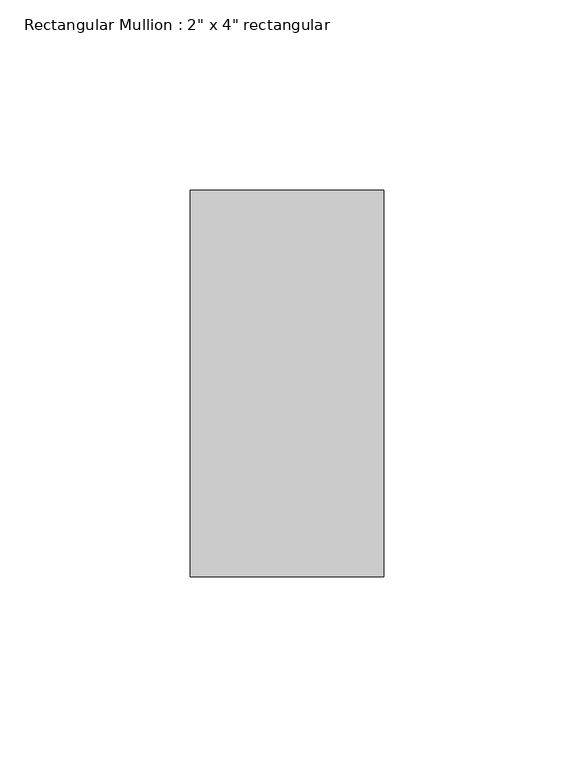
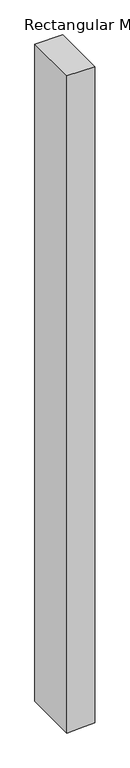
"""IFC4 building model written with IfcOpenShell, lengths in millimetres: member geometry."""

from ifc_helpers import new_model, si_unit, frame, origin, place, context, project, spatial, polyline, outline, extrude, source, transform, mapped, element, save


def member_64a94326(model_context):
    return source(origin(), model_context, "Body", "SweptSolid", [
        extrude(outline(polyline([(0.0, 25.4), (0.0, -25.4), (-1271.5510925, -25.4), (-1270.5808772, -2.1148317), (-1269.4344259, 25.4), (0.0, 25.4)])), frame((0.0, -50.8, 0.0), z_axis=(0.0, 1.0, 0.0), x_axis=(0.0, 0.0, 1.0)), (0.0, 0.0, 1.0), 101.6),
    ])


if __name__ == "__main__":
    model = new_model("IFC4")
    model_context = context("Model", 3, world=origin())
    ifc_project = project(units=[si_unit("LENGTHUNIT", "METRE", prefix="MILLI")], contexts=[model_context])
    site = spatial("IfcSite", under=ifc_project)
    building = spatial("IfcBuilding", under=site)
    placement = place(None, origin())
    member_shape = member_64a94326(model_context)
    element("IfcMember", 1, ObjectType="Rectangular Mullion : 2\" x 4\" rectangular", at=placement, inside=building, context=model_context, shape_type="MappedRepresentation", body=[
        mapped(member_shape, transform((0.0, 0.0, 0.0), x_axis=(1.0, 0.0, 0.0), y_axis=(0.0, 1.0, 0.0), z_axis=(0.0, 0.0, 1.0))),
    ])
    save(model, "model.ifc")

# Revit data of these elements
# Type "Rectangular Mullion : 2\" x 4\" rectangular"
#   built-in parameter 1007304 = 0.333333 (stored number, unit not read)
#   built-in parameter 1007301 = 0.0833333 (stored number, unit not read)
#   built-in parameter 1007300 = 0.0833333 (stored number, unit not read)
# Element 1 (IfcMember, "Rectangular Mullion : 2\" x 4\" rectangular")
#   Materials on its faces: "PAINTED STEEL C CHANNEL"
# Materials
#   "PAINTED STEEL C CHANNEL": class "Generic", colour RGB 88 62 61, transparency 0, Cost = 0
